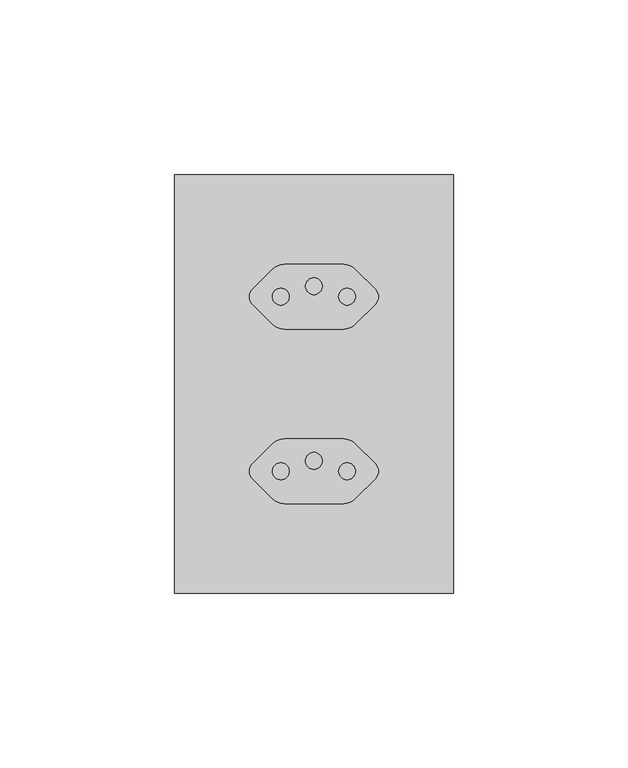
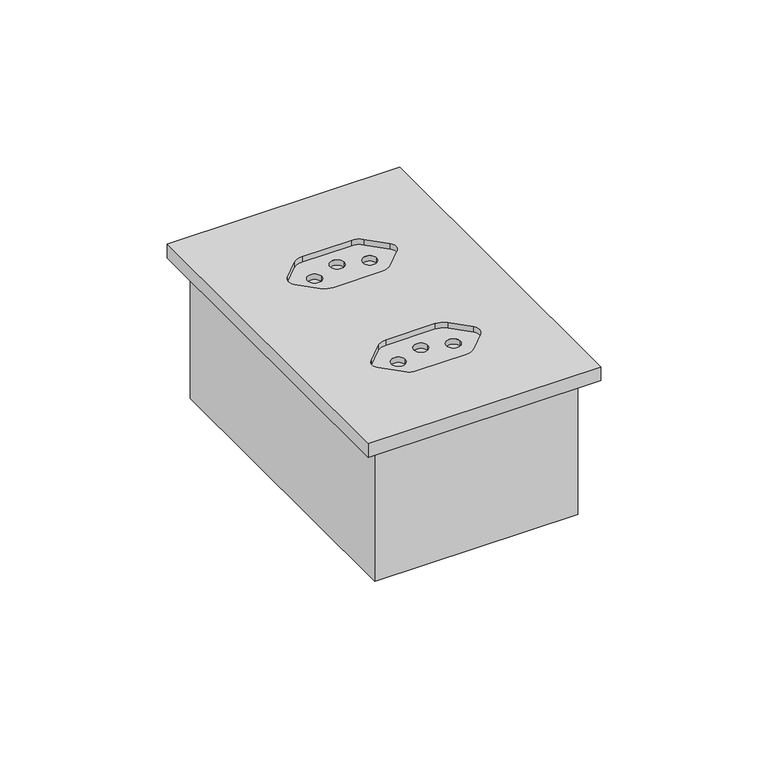
"""IFC4 building model written with IfcOpenShell, lengths in millimetres: proxy geometry, CAIXA VERTICE V7 : Tomada 20A 2s."""

import ifcopenshell
import ifcopenshell.guid

model = None  # the IFC model being written
_history = None  # IfcOwnerHistory: only IFC2X3 demands one
_inside = {}  # id of a spatial element -> (the spatial element, [elements in it])
_under = {}  # id of a project, library or spatial element -> (it, [spatial elements below it])
_declared = {}  # id of a project -> (the project, [libraries it declares])
_typed = {}  # id of a type object -> (the type object, [elements of that type])
_made_of = {}  # id of a material, layer set ... -> (it, [elements and type objects made of it])


def new_model(schema):
    """Start an empty IFC model of exactly this schema.

    Asked for "IFC4X3", IfcOpenShell would pick the latest addendum, in which some entities
    have other attributes; the version numbers below select the first issue.
    IFC2X3 requires an IfcOwnerHistory on every rooted entity: one is made here for all.
    """
    global model, _history
    if schema == "IFC4X3":
        model = ifcopenshell.file(schema_version=(4, 3, 0, 0))
    else:
        model = ifcopenshell.file(schema=schema)
    _inside.clear()
    _under.clear()
    _declared.clear()
    _typed.clear()
    _made_of.clear()
    _history = None
    if model.schema == "IFC2X3":
        org = make("IfcOrganization", Name="unknown")
        user = make(
            "IfcPersonAndOrganization",
            ThePerson=make("IfcPerson", FamilyName="unknown"),
            TheOrganization=org,
        )
        app = make(
            "IfcApplication",
            ApplicationDeveloper=org,
            Version="unknown",
            ApplicationFullName="unknown",
            ApplicationIdentifier="unknown",
        )
        _history = make(
            "IfcOwnerHistory",
            OwningUser=user,
            OwningApplication=app,
            ChangeAction="ADDED",
            CreationDate=0,
        )
    return model


def make(cls, **values):
    """One entity of the class cls with the attributes given. An attribute that is None is left unset."""
    return model.create_entity(
        cls, **{name: value for name, value in values.items() if value is not None}
    )


def rooted(cls, **values):
    """An entity with a GlobalId (a new one), such as an element, a storey or a relation."""
    return make(cls, GlobalId=ifcopenshell.guid.new(), OwnerHistory=_history, **values)


def si_unit(unit_type, name, prefix=None):
    """IfcSIUnit, for example si_unit("LENGTHUNIT", "METRE", prefix="MILLI")."""
    return make("IfcSIUnit", UnitType=unit_type, Prefix=prefix, Name=name)


def assignment(units):
    """IfcUnitAssignment: the units of a project."""
    return None if units is None else make("IfcUnitAssignment", Units=units)


def point(xyz):
    """IfcCartesianPoint."""
    return None if xyz is None else make("IfcCartesianPoint", Coordinates=xyz)


def direction(xyz):
    """IfcDirection."""
    return None if xyz is None else make("IfcDirection", DirectionRatios=xyz)


def frame(location, z_axis=None, x_axis=None):
    """IfcAxis2Placement3D, a coordinate frame: its origin and axes. An axis left out is left unset."""
    return make(
        "IfcAxis2Placement3D",
        Location=point(location),
        Axis=direction(z_axis),
        RefDirection=direction(x_axis),
    )


def origin():
    """The frame at (0, 0, 0) with its axes left unset."""
    return frame((0.0, 0.0, 0.0))


def place(relative_to, where):
    """IfcLocalPlacement: puts the frame where relative to a parent placement (None: the world)."""
    return make(
        "IfcLocalPlacement", PlacementRelTo=relative_to, RelativePlacement=where
    )


def context(
    kind, dimensions, precision=None, world=None, true_north=None, identifier=None
):
    """IfcGeometricRepresentationContext, for example the 3D "Model" context."""
    return make(
        "IfcGeometricRepresentationContext",
        ContextIdentifier=identifier,
        ContextType=kind,
        CoordinateSpaceDimension=dimensions,
        Precision=precision,
        WorldCoordinateSystem=world,
        TrueNorth=true_north,
    )


def project(units=None, contexts=None):
    """IfcProject with its units and contexts."""
    return rooted(
        "IfcProject",
        Name="project",
        RepresentationContexts=contexts,
        UnitsInContext=assignment(units),
    )


def spatial(cls, under=None, at=None, **own):
    """A site, building, storey or space (cls), placed at a placement, below another one or the project."""
    s = rooted(cls, ObjectPlacement=at, **own)
    if under is not None:
        _under.setdefault(under.id(), (under, []))[1].append(s)
    return s


def polyline(points):
    """IfcPolyline through the points."""
    return make("IfcPolyline", Points=[point(p) for p in points])


def circle_curve(where, radius):
    """IfcCircle in the frame where."""
    return make("IfcCircle", Position=where, Radius=radius)


def faces_of(points, faces, orient=None, outer=None):
    """IfcFace entities. A face is a list of loops; a loop is a list of indices into points, from 0.

    orient and outer hold one flag for each loop. By default every Orientation is true, the
    first loop of a face is its IfcFaceOuterBound and the others are IfcFaceBound.
    """
    made = []
    for i, loops in enumerate(faces):
        bounds = []
        for j, loop in enumerate(loops):
            is_outer = j == 0 if outer is None else outer[i][j]
            bounds.append(
                make(
                    "IfcFaceOuterBound" if is_outer else "IfcFaceBound",
                    Bound=make("IfcPolyLoop", Polygon=[points[k] for k in loop]),
                    Orientation=True if orient is None else orient[i][j],
                )
            )
        made.append(make("IfcFace", Bounds=bounds))
    return made


def faceted_brep(points, faces, orient=None, outer=None, voids=None):
    """IfcFacetedBrep: a solid bounded by flat faces; with voids (closed shells), ...WithVoids."""
    shared = [point(p) for p in points]
    hull = make("IfcClosedShell", CfsFaces=faces_of(shared, faces, orient, outer))
    if voids is None:
        return make("IfcFacetedBrep", Outer=hull)
    return make(
        "IfcFacetedBrepWithVoids",
        Outer=hull,
        Voids=[
            make(cls, CfsFaces=faces_of(shared, fs, o, b)) for cls, fs, o, b in voids
        ],
    )


def shape(context_of_items, identifier, shape_type, items):
    """IfcShapeRepresentation: the items that make up one representation, for example the "Body"."""
    return make(
        "IfcShapeRepresentation",
        ContextOfItems=context_of_items,
        RepresentationIdentifier=identifier,
        RepresentationType=shape_type,
        Items=items,
    )


def source(mapping_origin, context_of_items, identifier, shape_type, items):
    """IfcRepresentationMap: a shape defined once, which mapped items show again and again."""
    return make(
        "IfcRepresentationMap",
        MappingOrigin=mapping_origin,
        MappedRepresentation=shape(context_of_items, identifier, shape_type, items),
    )


def transform(
    local_origin,
    x_axis=None,
    y_axis=None,
    z_axis=None,
    scale=None,
    scale2=None,
    scale3=None,
    uniform=True,
):
    """IfcCartesianTransformationOperator3D, or its non-uniform kind. x_axis, y_axis, z_axis: its Axis1, 2, 3."""
    if uniform:
        return make(
            "IfcCartesianTransformationOperator3D",
            Axis1=direction(x_axis),
            Axis2=direction(y_axis),
            LocalOrigin=point(local_origin),
            Scale=scale,
            Axis3=direction(z_axis),
        )
    return make(
        "IfcCartesianTransformationOperator3DnonUniform",
        Axis1=direction(x_axis),
        Axis2=direction(y_axis),
        LocalOrigin=point(local_origin),
        Scale=scale,
        Axis3=direction(z_axis),
        Scale2=scale2,
        Scale3=scale3,
    )


def mapped(mapping_source, mapping_target):
    """IfcMappedItem: shows the shape of a source again, moved by a transform."""
    return make(
        "IfcMappedItem", MappingSource=mapping_source, MappingTarget=mapping_target
    )


def made_of(thing, what):
    """Note that an element or type object is made of a material, layer set ...; save() writes the relation."""
    if what is not None:
        _made_of.setdefault(what.id(), (what, []))[1].append(thing)
    return thing


def element(
    cls,
    number,
    at=None,
    inside=None,
    cuts=None,
    type_object=None,
    material=None,
    context=None,
    identifier="Body",
    shape_type=None,
    held_by="IfcProductDefinitionShape",
    body=None,
    shapes=None,
    **own,
):
    """One element of the class cls, such as IfcWall. Its Tag is "e" and its number.

    at: its placement. inside: the storey or other place that contains it. cuts: it is an
    opening in that element (IfcRelVoidsElement). A single representation is given by context,
    identifier, shape_type and body (its items); several are given by shapes. held_by: the class
    of the entity that holds the representations. save() writes the other relations.
    """
    e = rooted(cls, Tag="e%d" % number, ObjectPlacement=at, **own)
    if body is not None:
        shapes = [shape(context, identifier, shape_type, body)]
    if shapes is not None:
        e.Representation = make(held_by, Representations=shapes)
    if inside is not None:
        _inside.setdefault(inside.id(), (inside, []))[1].append(e)
    if cuts is not None:
        rooted(
            "IfcRelVoidsElement", RelatingBuildingElement=cuts, RelatedOpeningElement=e
        )
    if type_object is not None:
        _typed.setdefault(type_object.id(), (type_object, []))[1].append(e)
    return made_of(e, material)


def aggregate(whole, parts):
    """IfcRelAggregates: a whole, such as a stair, and the parts it consists of."""
    return rooted("IfcRelAggregates", RelatingObject=whole, RelatedObjects=parts)


def save(model, path):
    """Write the relations noted so far, then the file.

    IfcRelAggregates (storeys below a building ...), IfcRelContainedInSpatialStructure (elements
    in a storey), IfcRelDefinesByType, IfcRelAssociatesMaterial and IfcRelDeclares: one each for
    every whole, place, type object, material and project.
    """
    for whole, parts in _under.values():
        aggregate(whole, parts)
    for where, things in _inside.values():
        rooted(
            "IfcRelContainedInSpatialStructure",
            RelatedElements=things,
            RelatingStructure=where,
        )
    for kind, things in _typed.values():
        rooted("IfcRelDefinesByType", RelatedObjects=things, RelatingType=kind)
    for what, things in _made_of.values():
        rooted("IfcRelAssociatesMaterial", RelatedObjects=things, RelatingMaterial=what)
    for by, libraries in _declared.values():
        rooted("IfcRelDeclares", RelatingContext=by, RelatedDefinitions=libraries)
    model.write(path)


def plane_surface(at):
    """IfcPlane: the flat surface through the origin of the frame at, square to its z axis."""
    return make("IfcPlane", Position=at)


def revolved_surface(curve, axis_point, axis_direction):
    """IfcSurfaceOfRevolution: the curve turned about the line through axis_point along axis_direction."""
    return make(
        "IfcSurfaceOfRevolution",
        SweptCurve=make("IfcArbitraryOpenProfileDef", ProfileType="CURVE", Curve=curve),
        AxisPosition=make("IfcAxis1Placement", Location=point(axis_point), Axis=direction(axis_direction)),
    )


def advanced_brep(points, edges, surfaces, faces):
    """IfcAdvancedBrep: a solid bounded by faces that lie on surfaces and meet in shared edges.

    An edge is (start, end): straight between two places in points (the first is 0);
    or (start, end, curve); or (start, end, curve, False) where it runs against its curve.
    A face is (place in surfaces, loops), or (place, loops, False) where it looks against
    its surface's normal. A loop lists edges by number (the first is 1), with a minus sign
    where the edge is run from its end to its start. The first loop is the outer one.
    """
    corners = [point(p) for p in points]
    vertices = [make("IfcVertexPoint", VertexGeometry=c) for c in corners]
    made = []
    for start, end, *more in edges:
        made.append(
            make(
                "IfcEdgeCurve",
                EdgeStart=vertices[start],
                EdgeEnd=vertices[end],
                EdgeGeometry=more[0] if more else make("IfcPolyline", Points=[corners[start], corners[end]]),
                SameSense=more[1] if len(more) > 1 else True,
            )
        )
    hull = []
    for where, loops, *sense in faces:
        bounds = []
        for j, loop in enumerate(loops):
            ring = [make("IfcOrientedEdge", EdgeElement=made[abs(k) - 1], Orientation=k > 0) for k in loop]
            bounds.append(
                make(
                    "IfcFaceOuterBound" if j == 0 else "IfcFaceBound",
                    Bound=make("IfcEdgeLoop", EdgeList=ring),
                    Orientation=True,
                )
            )
        hull.append(make("IfcAdvancedFace", Bounds=bounds, FaceSurface=surfaces[where], SameSense=sense[0] if sense else True))
    return make("IfcAdvancedBrep", Outer=make("IfcClosedShell", CfsFaces=hull))


def electrical_fixtures_32f15f6c(model_context):
    return source(origin(), model_context, "Body", "SolidModel", [
        faceted_brep([(33.0, 1047.0, -48.0), (33.0, 1153.0, -48.0), (-33.0, 1153.0, -48.0), (-33.0, 1047.0, -48.0), (35.0, 1155.0, -50.0), (35.0, 1045.0, -50.0), (-35.0, 1045.0, -50.0), (-35.0, 1155.0, -50.0), (-35.0, 1155.0, 0.0), (35.0, 1155.0, 0.0), (-35.0, 1045.0, 0.0), (35.0, 1045.0, 0.0), (33.0, 1153.0, 0.0), (33.0, 1047.0, 0.0), (-33.0, 1047.0, 0.0), (-33.0, 1153.0, 0.0)], [[[0, 1, 2, 3]], [[4, 5, 6, 7]], [[4, 7, 8, 9]], [[8, 7, 6, 10]], [[10, 6, 5, 11]], [[11, 5, 4, 9]], [[9, 8, 10, 11], [12, 13, 14, 15]], [[13, 12, 1, 0]], [[14, 13, 0, 3]], [[15, 14, 3, 2]], [[12, 15, 2, 1]]]),
        advanced_brep(
        [(40.0, 1160.0, 5.0), (-40.0, 1160.0, 5.0), (-40.0, 1040.0, 5.0), (40.0, 1040.0, 5.0), (8.4215729, 1115.75, 5.0), (-8.4215729, 1115.75, 5.0), (-11.9571068, 1117.2144661, 5.0), (-17.6213203, 1122.8786797, 5.0), (-17.6213203, 1127.1213203, 5.0), (-11.9571068, 1132.7855339, 5.0), (-8.4215729, 1134.25, 5.0), (8.4215729, 1134.25, 5.0), (11.9571068, 1132.7855339, 5.0), (17.6213203, 1127.1213203, 5.0), (17.6213203, 1122.8786797, 5.0), (11.9571068, 1117.2144661, 5.0), (8.4215729, 1065.75, 5.0), (-8.4215729, 1065.75, 5.0), (-11.9571068, 1067.2144661, 5.0), (-17.6213203, 1072.8786797, 5.0), (-17.6213203, 1077.1213203, 5.0), (-11.9571068, 1082.7855339, 5.0), (-8.4215729, 1084.25, 5.0), (8.4215729, 1084.25, 5.0), (11.9571068, 1082.7855339, 5.0), (17.6213203, 1077.1213203, 5.0), (17.6213203, 1072.8786797, 5.0), (11.9571068, 1067.2144661, 5.0), (-40.0, 1160.0, 0.0), (40.0, 1160.0, 0.0), (40.0, 1040.0, 0.0), (-40.0, 1040.0, 0.0), (8.4215729, 1115.75, 3.0), (11.9571068, 1117.2144661, 3.0), (17.6213203, 1122.8786797, 3.0), (17.6213203, 1127.1213203, 3.0), (11.9571068, 1132.7855339, 3.0), (8.4215729, 1134.25, 3.0), (-8.4215729, 1134.25, 3.0), (-11.9571068, 1132.7855339, 3.0), (-17.6213203, 1127.1213203, 3.0), (-17.6213203, 1122.8786797, 3.0), (-11.9571068, 1117.2144661, 3.0), (-8.4215729, 1115.75, 3.0), (-7.1, 1125.0, 3.0), (-11.9, 1125.0, 3.0), (11.9, 1125.0, 3.0), (7.1, 1125.0, 3.0), (2.4, 1128.0, 3.0), (-2.4, 1128.0, 3.0), (-11.9, 1125.0, 1.0), (-7.1, 1125.0, 1.0), (7.1, 1125.0, 1.0), (11.9, 1125.0, 1.0), (-2.4, 1128.0, 1.0), (2.4, 1128.0, 1.0), (8.4215729, 1065.75, 3.0), (11.9571068, 1067.2144661, 3.0), (17.6213203, 1072.8786797, 3.0), (17.6213203, 1077.1213203, 3.0), (11.9571068, 1082.7855339, 3.0), (8.4215729, 1084.25, 3.0), (-8.4215729, 1084.25, 3.0), (-11.9571068, 1082.7855339, 3.0), (-17.6213203, 1077.1213203, 3.0), (-17.6213203, 1072.8786797, 3.0), (-11.9571068, 1067.2144661, 3.0), (-8.4215729, 1065.75, 3.0), (-7.1, 1075.0, 3.0), (-11.9, 1075.0, 3.0), (11.9, 1075.0, 3.0), (7.1, 1075.0, 3.0), (2.4, 1078.0, 3.0), (-2.4, 1078.0, 3.0), (-11.9, 1075.0, 1.0), (-7.1, 1075.0, 1.0), (7.1, 1075.0, 1.0), (11.9, 1075.0, 1.0), (-2.4, 1078.0, 1.0), (2.4, 1078.0, 1.0)],
        [
            (0, 1),
            (1, 2),
            (2, 3),
            (3, 0),
            (4, 5),
            (5, 6, circle_curve(frame((-8.4215729, 1120.75, 5.0), z_axis=(0.0, 0.0, -1.0), x_axis=(-1.0, 0.0, 0.0)), 5.0)),
            (6, 7),
            (7, 8, circle_curve(frame((-15.5, 1125.0, 5.0), z_axis=(0.0, 0.0, -1.0), x_axis=(-1.0, 0.0, 0.0)), 3.0)),
            (8, 9),
            (9, 10, circle_curve(frame((-8.4215729, 1129.25, 5.0), z_axis=(0.0, 0.0, -1.0), x_axis=(-1.0, 0.0, 0.0)), 5.0)),
            (10, 11),
            (11, 12, circle_curve(frame((8.4215729, 1129.25, 5.0), z_axis=(0.0, 0.0, -1.0), x_axis=(-1.0, 0.0, 0.0)), 5.0)),
            (12, 13),
            (13, 14, circle_curve(frame((15.5, 1125.0, 5.0), z_axis=(0.0, 0.0, -1.0), x_axis=(-1.0, 0.0, 0.0)), 3.0)),
            (14, 15),
            (15, 4, circle_curve(frame((8.4215729, 1120.75, 5.0), z_axis=(0.0, 0.0, -1.0), x_axis=(-1.0, 0.0, 0.0)), 5.0)),
            (16, 17),
            (17, 18, circle_curve(frame((-8.4215729, 1070.75, 5.0), z_axis=(0.0, 0.0, -1.0), x_axis=(-1.0, 0.0, 0.0)), 5.0)),
            (18, 19),
            (19, 20, circle_curve(frame((-15.5, 1075.0, 5.0), z_axis=(0.0, 0.0, -1.0), x_axis=(-1.0, 0.0, 0.0)), 3.0)),
            (20, 21),
            (21, 22, circle_curve(frame((-8.4215729, 1079.25, 5.0), z_axis=(0.0, 0.0, -1.0), x_axis=(-1.0, 0.0, 0.0)), 5.0)),
            (22, 23),
            (23, 24, circle_curve(frame((8.4215729, 1079.25, 5.0), z_axis=(0.0, 0.0, -1.0), x_axis=(-1.0, 0.0, 0.0)), 5.0)),
            (24, 25),
            (25, 26, circle_curve(frame((15.5, 1075.0, 5.0), z_axis=(0.0, 0.0, -1.0), x_axis=(-1.0, 0.0, 0.0)), 3.0)),
            (26, 27),
            (27, 16, circle_curve(frame((8.4215729, 1070.75, 5.0), z_axis=(0.0, 0.0, -1.0), x_axis=(-1.0, 0.0, 0.0)), 5.0)),
            (28, 29),
            (29, 30),
            (30, 31),
            (31, 28),
            (0, 29),
            (28, 1),
            (31, 2),
            (30, 3),
            (32, 33, circle_curve(frame((8.4215729, 1120.75, 3.0), z_axis=(0.0, 0.0, 1.0), x_axis=(-1.0, 0.0, 0.0)), 5.0)),
            (33, 34),
            (34, 35, circle_curve(frame((15.5, 1125.0, 3.0), z_axis=(0.0, 0.0, 1.0), x_axis=(-1.0, 0.0, 0.0)), 3.0)),
            (35, 36),
            (36, 37, circle_curve(frame((8.4215729, 1129.25, 3.0), z_axis=(0.0, 0.0, 1.0), x_axis=(-1.0, 0.0, 0.0)), 5.0)),
            (37, 38),
            (38, 39, circle_curve(frame((-8.4215729, 1129.25, 3.0), z_axis=(0.0, 0.0, 1.0), x_axis=(-1.0, 0.0, 0.0)), 5.0)),
            (39, 40),
            (40, 41, circle_curve(frame((-15.5, 1125.0, 3.0), z_axis=(0.0, 0.0, 1.0), x_axis=(-1.0, 0.0, 0.0)), 3.0)),
            (41, 42),
            (42, 43, circle_curve(frame((-8.4215729, 1120.75, 3.0), z_axis=(0.0, 0.0, 1.0), x_axis=(-1.0, 0.0, 0.0)), 5.0)),
            (43, 32),
            (44, 45, circle_curve(frame((-9.5, 1125.0, 3.0), z_axis=(0.0, 0.0, -1.0), x_axis=(1.0, 2.301812013077709e-12, 0.0)), 2.4)),
            (45, 44, circle_curve(frame((-9.5, 1125.0, 3.0), z_axis=(0.0, 0.0, -1.0), x_axis=(1.0, 2.301812013077709e-12, 0.0)), 2.4)),
            (46, 47, circle_curve(frame((9.5, 1125.0, 3.0), z_axis=(0.0, 0.0, -1.0), x_axis=(1.0, 2.301812013077709e-12, 0.0)), 2.4)),
            (47, 46, circle_curve(frame((9.5, 1125.0, 3.0), z_axis=(0.0, 0.0, -1.0), x_axis=(1.0, 2.301812013077709e-12, 0.0)), 2.4)),
            (48, 49, circle_curve(frame((0.0, 1128.0, 3.0), z_axis=(0.0, 0.0, -1.0), x_axis=(1.0, 2.301812013077709e-12, 0.0)), 2.4)),
            (49, 48, circle_curve(frame((0.0, 1128.0, 3.0), z_axis=(0.0, 0.0, -1.0), x_axis=(1.0, 2.301812013077709e-12, 0.0)), 2.4)),
            (43, 5),
            (4, 32),
            (42, 6),
            (41, 7),
            (40, 8),
            (39, 9),
            (38, 10),
            (37, 11),
            (36, 12),
            (35, 13),
            (34, 14),
            (33, 15),
            (50, 51, circle_curve(frame((-9.5, 1125.0, 1.0), z_axis=(0.0, 0.0, 1.0), x_axis=(1.0, 2.301812013077709e-12, 0.0)), 2.4)),
            (51, 50, circle_curve(frame((-9.5, 1125.0, 1.0), z_axis=(0.0, 0.0, 1.0), x_axis=(1.0, 2.301812013077709e-12, 0.0)), 2.4)),
            (52, 53, circle_curve(frame((9.5, 1125.0, 1.0), z_axis=(0.0, 0.0, 1.0), x_axis=(1.0, 2.301812013077709e-12, 0.0)), 2.4)),
            (53, 52, circle_curve(frame((9.5, 1125.0, 1.0), z_axis=(0.0, 0.0, 1.0), x_axis=(1.0, 2.301812013077709e-12, 0.0)), 2.4)),
            (54, 55, circle_curve(frame((0.0, 1128.0, 1.0), z_axis=(0.0, 0.0, 1.0), x_axis=(1.0, 2.301812013077709e-12, 0.0)), 2.4)),
            (55, 54, circle_curve(frame((0.0, 1128.0, 1.0), z_axis=(0.0, 0.0, 1.0), x_axis=(1.0, 2.301812013077709e-12, 0.0)), 2.4)),
            (44, 51),
            (50, 45),
            (46, 53),
            (52, 47),
            (48, 55),
            (54, 49),
            (56, 57, circle_curve(frame((8.4215729, 1070.75, 3.0), z_axis=(0.0, 0.0, 1.0), x_axis=(-1.0, 0.0, 0.0)), 5.0)),
            (57, 58),
            (58, 59, circle_curve(frame((15.5, 1075.0, 3.0), z_axis=(0.0, 0.0, 1.0), x_axis=(-1.0, 0.0, 0.0)), 3.0)),
            (59, 60),
            (60, 61, circle_curve(frame((8.4215729, 1079.25, 3.0), z_axis=(0.0, 0.0, 1.0), x_axis=(-1.0, 0.0, 0.0)), 5.0)),
            (61, 62),
            (62, 63, circle_curve(frame((-8.4215729, 1079.25, 3.0), z_axis=(0.0, 0.0, 1.0), x_axis=(-1.0, 0.0, 0.0)), 5.0)),
            (63, 64),
            (64, 65, circle_curve(frame((-15.5, 1075.0, 3.0), z_axis=(0.0, 0.0, 1.0), x_axis=(-1.0, 0.0, 0.0)), 3.0)),
            (65, 66),
            (66, 67, circle_curve(frame((-8.4215729, 1070.75, 3.0), z_axis=(0.0, 0.0, 1.0), x_axis=(-1.0, 0.0, 0.0)), 5.0)),
            (67, 56),
            (68, 69, circle_curve(frame((-9.5, 1075.0, 3.0), z_axis=(0.0, 0.0, -1.0), x_axis=(1.0, 2.301812013077709e-12, 0.0)), 2.4)),
            (69, 68, circle_curve(frame((-9.5, 1075.0, 3.0), z_axis=(0.0, 0.0, -1.0), x_axis=(1.0, 2.301812013077709e-12, 0.0)), 2.4)),
            (70, 71, circle_curve(frame((9.5, 1075.0, 3.0), z_axis=(0.0, 0.0, -1.0), x_axis=(1.0, 2.301812013077709e-12, 0.0)), 2.4)),
            (71, 70, circle_curve(frame((9.5, 1075.0, 3.0), z_axis=(0.0, 0.0, -1.0), x_axis=(1.0, 2.301812013077709e-12, 0.0)), 2.4)),
            (72, 73, circle_curve(frame((0.0, 1078.0, 3.0), z_axis=(0.0, 0.0, -1.0), x_axis=(1.0, 2.301812013077709e-12, 0.0)), 2.4)),
            (73, 72, circle_curve(frame((0.0, 1078.0, 3.0), z_axis=(0.0, 0.0, -1.0), x_axis=(1.0, 2.301812013077709e-12, 0.0)), 2.4)),
            (67, 17),
            (16, 56),
            (66, 18),
            (65, 19),
            (64, 20),
            (63, 21),
            (62, 22),
            (61, 23),
            (60, 24),
            (59, 25),
            (58, 26),
            (57, 27),
            (74, 75, circle_curve(frame((-9.5, 1075.0, 1.0), z_axis=(0.0, 0.0, 1.0), x_axis=(1.0, 2.301812013077709e-12, 0.0)), 2.4)),
            (75, 74, circle_curve(frame((-9.5, 1075.0, 1.0), z_axis=(0.0, 0.0, 1.0), x_axis=(1.0, 2.301812013077709e-12, 0.0)), 2.4)),
            (76, 77, circle_curve(frame((9.5, 1075.0, 1.0), z_axis=(0.0, 0.0, 1.0), x_axis=(1.0, 2.301812013077709e-12, 0.0)), 2.4)),
            (77, 76, circle_curve(frame((9.5, 1075.0, 1.0), z_axis=(0.0, 0.0, 1.0), x_axis=(1.0, 2.301812013077709e-12, 0.0)), 2.4)),
            (78, 79, circle_curve(frame((0.0, 1078.0, 1.0), z_axis=(0.0, 0.0, 1.0), x_axis=(1.0, 2.301812013077709e-12, 0.0)), 2.4)),
            (79, 78, circle_curve(frame((0.0, 1078.0, 1.0), z_axis=(0.0, 0.0, 1.0), x_axis=(1.0, 2.301812013077709e-12, 0.0)), 2.4)),
            (68, 75),
            (74, 69),
            (70, 77),
            (76, 71),
            (72, 79),
            (78, 73),
        ],
        [
            plane_surface(frame((-60.0, 1160.0, 5.0), z_axis=(0.0, 0.0, 1.0), x_axis=(-1.0, 0.0, 0.0))),
            plane_surface(frame((-60.0, 1160.0, 0.0), z_axis=(0.0, 0.0, -1.0), x_axis=(1.0, 0.0, 0.0))),
            plane_surface(frame((40.0, 1160.0, 5.0), z_axis=(0.0, 1.0, 0.0), x_axis=(0.0, 0.0, -1.0))),
            plane_surface(frame((-40.0, 1160.0, 5.0), z_axis=(-1.0, 0.0, 0.0), x_axis=(0.0, 0.0, -1.0))),
            plane_surface(frame((-40.0, 1040.0, 5.0), z_axis=(0.0, -1.0, 0.0), x_axis=(0.0, 0.0, -1.0))),
            plane_surface(frame((40.0, 1040.0, 5.0), z_axis=(1.0, 0.0, 0.0), x_axis=(0.0, 0.0, -1.0))),
            plane_surface(frame((3.4215729, 1120.75, 3.0), z_axis=(0.0, 0.0, 1.0), x_axis=(0.0, 1.0, 0.0))),
            plane_surface(frame((-8.4215729, 1115.75, 5.0), z_axis=(0.0, 1.0, 0.0), x_axis=(0.0, 0.0, -1.0))),
            revolved_surface(polyline([(-13.4215729, 1120.75, 5.0), (-13.4215729, 1120.75, 3.0)]), (-8.4215729, 1120.75, 3.0), (0.0, 0.0, 1.0)),
            plane_surface(frame((-17.6213203, 1122.8786797, 5.0), z_axis=(0.7071067811865045, 0.7071067811865905, 0.0), x_axis=(0.0, 0.0, -1.0))),
            revolved_surface(polyline([(-18.5, 1125.0, 5.0), (-18.5, 1125.0, 3.0)]), (-15.5, 1125.0, 3.0), (0.0, 0.0, 1.0)),
            plane_surface(frame((-11.9571068, 1132.7855339, 5.0), z_axis=(0.7071067811865515, -0.7071067811865437, 0.0), x_axis=(0.0, 0.0, -1.0))),
            revolved_surface(polyline([(-13.4215729, 1129.25, 5.0), (-13.4215729, 1129.25, 3.0)]), (-8.4215729, 1129.25, 3.0), (0.0, 0.0, 1.0)),
            plane_surface(frame((8.4215729, 1134.25, 5.0), z_axis=(0.0, -1.0, 0.0), x_axis=(0.0, 0.0, -1.0))),
            revolved_surface(polyline([(3.4215728999999993, 1129.25, 5.0), (3.4215728999999993, 1129.25, 3.0)]), (8.4215729, 1129.25, 3.0), (0.0, 0.0, 1.0)),
            plane_surface(frame((17.6213203, 1127.1213203, 5.0), z_axis=(-0.7071067811865307, -0.7071067811865643, 0.0), x_axis=(0.0, 0.0, -1.0))),
            revolved_surface(polyline([(12.5, 1125.0, 5.0), (12.5, 1125.0, 3.0)]), (15.5, 1125.0, 3.0), (0.0, 0.0, 1.0)),
            plane_surface(frame((11.9571068, 1117.2144661, 5.0), z_axis=(-0.7071067811865893, 0.7071067811865058, 0.0), x_axis=(0.0, 0.0, -1.0))),
            revolved_surface(polyline([(3.4215728999999993, 1120.75, 5.0), (3.4215728999999993, 1120.75, 3.0)]), (8.4215729, 1120.75, 3.0), (0.0, 0.0, 1.0)),
            plane_surface(frame((-7.1, 1125.0, 1.0), z_axis=(0.0, 0.0, 1.0), x_axis=(2.301812013077709e-12, -1.0, 0.0))),
            revolved_surface(polyline([(-7.1, 1125.0000000000055, 3.0), (-7.1, 1125.0000000000055, 1.0)]), (-9.5, 1125.0, 1.0), (0.0, 0.0, 1.0)),
            revolved_surface(polyline([(11.9, 1125.0000000000055, 3.0), (11.9, 1125.0000000000055, 1.0)]), (9.5, 1125.0, 5.0), (0.0, 0.0, 1.0)),
            revolved_surface(polyline([(2.4, 1128.0000000000055, 3.0), (2.4, 1128.0000000000055, 1.0)]), (0.0, 1128.0, 5.0), (0.0, 0.0, 1.0)),
            plane_surface(frame((3.4215729, 1070.75, 3.0), z_axis=(0.0, 0.0, 1.0), x_axis=(0.0, 1.0, 0.0))),
            plane_surface(frame((-8.4215729, 1065.75, 5.0), z_axis=(0.0, 1.0, 0.0), x_axis=(0.0, 0.0, -1.0))),
            revolved_surface(polyline([(-13.4215729, 1070.75, 5.0), (-13.4215729, 1070.75, 3.0)]), (-8.4215729, 1070.75, 3.0), (0.0, 0.0, 1.0)),
            plane_surface(frame((-17.6213203, 1072.8786797, 5.0), z_axis=(0.7071067811865045, 0.7071067811865905, 0.0), x_axis=(0.0, 0.0, -1.0))),
            revolved_surface(polyline([(-18.5, 1075.0, 5.0), (-18.5, 1075.0, 3.0)]), (-15.5, 1075.0, 3.0), (0.0, 0.0, 1.0)),
            plane_surface(frame((-11.9571068, 1082.7855339, 5.0), z_axis=(0.7071067811865515, -0.7071067811865437, 0.0), x_axis=(0.0, 0.0, -1.0))),
            revolved_surface(polyline([(-13.4215729, 1079.25, 5.0), (-13.4215729, 1079.25, 3.0)]), (-8.4215729, 1079.25, 3.0), (0.0, 0.0, 1.0)),
            plane_surface(frame((8.4215729, 1084.25, 5.0), z_axis=(0.0, -1.0, 0.0), x_axis=(0.0, 0.0, -1.0))),
            revolved_surface(polyline([(3.4215728999999993, 1079.25, 5.0), (3.4215728999999993, 1079.25, 3.0)]), (8.4215729, 1079.25, 3.0), (0.0, 0.0, 1.0)),
            plane_surface(frame((17.6213203, 1077.1213203, 5.0), z_axis=(-0.7071067811865307, -0.7071067811865643, 0.0), x_axis=(0.0, 0.0, -1.0))),
            revolved_surface(polyline([(12.5, 1075.0, 5.0), (12.5, 1075.0, 3.0)]), (15.5, 1075.0, 3.0), (0.0, 0.0, 1.0)),
            plane_surface(frame((11.9571068, 1067.2144661, 5.0), z_axis=(-0.7071067811865893, 0.7071067811865058, 0.0), x_axis=(0.0, 0.0, -1.0))),
            revolved_surface(polyline([(3.4215728999999993, 1070.75, 5.0), (3.4215728999999993, 1070.75, 3.0)]), (8.4215729, 1070.75, 3.0), (0.0, 0.0, 1.0)),
            plane_surface(frame((-7.1, 1075.0, 1.0), z_axis=(0.0, 0.0, 1.0), x_axis=(2.301812013077709e-12, -1.0, 0.0))),
            revolved_surface(polyline([(-7.1, 1075.0000000000055, 3.0), (-7.1, 1075.0000000000055, 1.0)]), (-9.5, 1075.0, 1.0), (0.0, 0.0, 1.0)),
            revolved_surface(polyline([(11.9, 1075.0000000000055, 3.0), (11.9, 1075.0000000000055, 1.0)]), (9.5, 1075.0, 5.0), (0.0, 0.0, 1.0)),
            revolved_surface(polyline([(2.4, 1078.0000000000055, 3.0), (2.4, 1078.0000000000055, 1.0)]), (0.0, 1078.0, 5.0), (0.0, 0.0, 1.0)),
        ],
        [
            (0, [[1, 2, 3, 4], [5, 6, 7, 8, 9, 10, 11, 12, 13, 14, 15, 16], [17, 18, 19, 20, 21, 22, 23, 24, 25, 26, 27, 28]]),
            (1, [[29, 30, 31, 32]]),
            (2, [[-1, 33, -29, 34]]),
            (3, [[-2, -34, -32, 35]]),
            (4, [[-3, -35, -31, 36]]),
            (5, [[-4, -36, -30, -33]]),
            (6, [[37, 38, 39, 40, 41, 42, 43, 44, 45, 46, 47, 48], [49, 50], [51, 52], [53, 54]]),
            (7, [[-48, 55, -5, 56]]),
            (8, [[-47, 57, -6, -55]]),
            (9, [[-46, 58, -7, -57]]),
            (10, [[-45, 59, -8, -58]]),
            (11, [[-44, 60, -9, -59]]),
            (12, [[-43, 61, -10, -60]]),
            (13, [[-42, 62, -11, -61]]),
            (14, [[-41, 63, -12, -62]]),
            (15, [[-40, 64, -13, -63]]),
            (16, [[-39, 65, -14, -64]]),
            (17, [[-38, 66, -15, -65]]),
            (18, [[-37, -56, -16, -66]]),
            (19, [[67, 68]]),
            (19, [[69, 70]]),
            (19, [[71, 72]]),
            (20, [[-49, 73, -67, 74]]),
            (20, [[-50, -74, -68, -73]]),
            (21, [[-51, 75, -69, 76]]),
            (21, [[-52, -76, -70, -75]]),
            (22, [[-53, 77, -71, 78]]),
            (22, [[-54, -78, -72, -77]]),
            (23, [[79, 80, 81, 82, 83, 84, 85, 86, 87, 88, 89, 90], [91, 92], [93, 94], [95, 96]]),
            (24, [[-90, 97, -17, 98]]),
            (25, [[-89, 99, -18, -97]]),
            (26, [[-88, 100, -19, -99]]),
            (27, [[-87, 101, -20, -100]]),
            (28, [[-86, 102, -21, -101]]),
            (29, [[-85, 103, -22, -102]]),
            (30, [[-84, 104, -23, -103]]),
            (31, [[-83, 105, -24, -104]]),
            (32, [[-82, 106, -25, -105]]),
            (33, [[-81, 107, -26, -106]]),
            (34, [[-80, 108, -27, -107]]),
            (35, [[-79, -98, -28, -108]]),
            (36, [[109, 110]]),
            (36, [[111, 112]]),
            (36, [[113, 114]]),
            (37, [[-91, 115, -109, 116]]),
            (37, [[-92, -116, -110, -115]]),
            (38, [[-93, 117, -111, 118]]),
            (38, [[-94, -118, -112, -117]]),
            (39, [[-95, 119, -113, 120]]),
            (39, [[-96, -120, -114, -119]]),
        ],
    ),
    ])


if __name__ == "__main__":
    model = new_model("IFC4")
    model_context = context("Model", 3, world=origin())
    ifc_project = project(units=[si_unit("LENGTHUNIT", "METRE", prefix="MILLI")], contexts=[model_context])
    site = spatial("IfcSite", under=ifc_project)
    building = spatial("IfcBuilding", under=site)
    placement = place(None, origin())
    electrical_fixtures_shape = electrical_fixtures_32f15f6c(model_context)
    element("IfcBuildingElementProxy", 1, Name="CAIXA VERTICE V7 : Tomada 20A 2s", ObjectType="CAIXA VERTICE V7 : Tomada 20A 2s", at=placement, inside=building, context=model_context, shape_type="MappedRepresentation", body=[
        mapped(electrical_fixtures_shape, transform((0.0, 0.0, 0.0), x_axis=(1.0, 0.0, 0.0), y_axis=(0.0, 1.0, 0.0), z_axis=(0.0, 0.0, 1.0))),
    ])
    save(model, "model.ifc")

# Revit data of these elements
# Type "CAIXA VERTICE V7 : Tomada 20A 2s"
#   URL = "www.facebook.com/verticetreinamentos"
#   SEÇÃO [instance default] = ""
#   Rotação [instance default] = 0.00°
#   LARGURA DA TAMPA = 0.08 m
#   BORDA = 0.01 m
#   ALTURA DE INSTALAÇÃO [instance default] = 1.10 m
#   Distância Anotação [instance default] = 0.0015 m
#   ALTURA DA TAMPA = 0.12 m
#   Vertical [instance default] = yes
#   VER SEÇÃO [instance default] = no
#   SHADE ESQ [instance default] = no
#   SHADE DIR [instance default] = yes
#   HORIZONTAL [instance default] = no
#   ANDAR COM A LEGENDA [instance default] = 0
#   Material Tampa [instance default] = Plástico, branco opaco
#   Caixa = element 1798518
#   Anotação = element 1798532
#   Default Elevation = 0
# Element 1 (IfcBuildingElementProxy, "CAIXA VERTICE V7 : Tomada 20A 2s")
#   VER SEÇÃO = yes
#   Materials on its faces: "Plástico, branco opaco"
# Materials
#   "Plástico, branco opaco": class "Plástico", colour RGB 120 120 120, transparency 0, Description = "Plastic, generic, opaque white", Cost = 0
